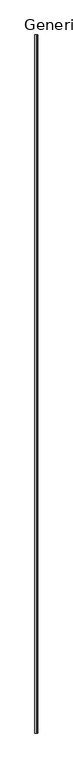
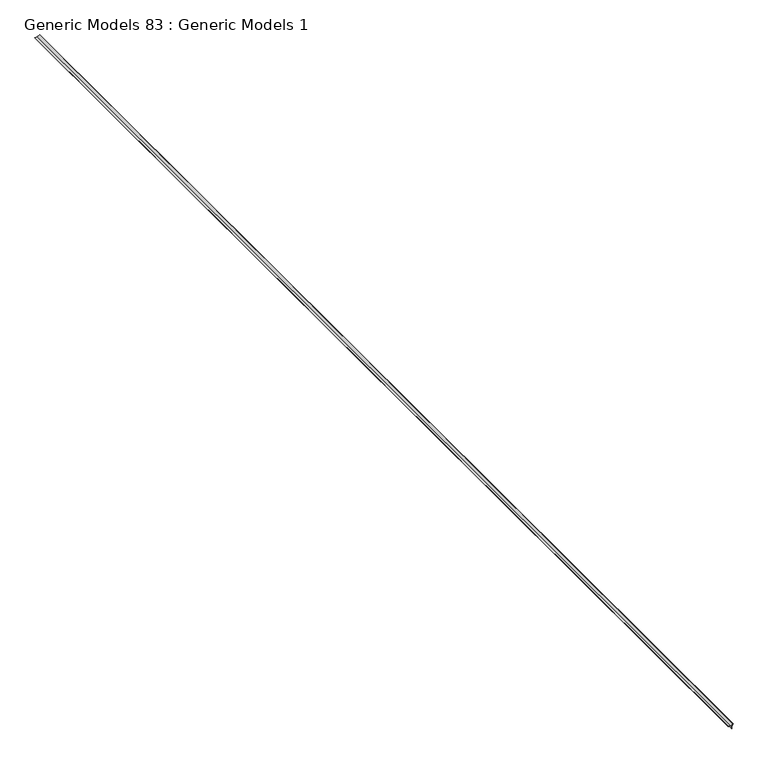
"""IFC4 building model written with IfcOpenShell, lengths in millimetres: proxy geometry, Generic Models 83 : Generic Models 1."""

from ifc_helpers import new_model, si_unit, point, frame, frame_2d, origin, place, context, project, spatial, polyline, circle_curve, trimmed, segment, composite_curve, outline, extrude, source, transform, mapped, element, save


def generic_models_83_generic_models_1_05889233(model_context):
    return source(origin(), model_context, "Body", "SweptSolid", [
        extrude(outline(composite_curve([segment(polyline([(127128.4926156, 9702.5518851), (127108.966, 9664.5263704), (127108.966, 9626.4263704), (127107.696, 9626.4263704), (127107.696, 9664.8333942), (127127.5962396, 9703.5864924), (127088.8431414, 9683.6862528), (127050.4361176, 9683.6862528), (127050.4361176, 9684.9562528), (127088.5361176, 9684.9562528), (127126.5616323, 9704.4828684)]), True, "CONTINUOUS"), segment(trimmed(circle_curve(frame_2d((127127.2167873, 9703.2070401)), 1.4342127), [point((127126.5616323, 9704.4828684))], [point((127128.4926156, 9702.5518851))], False, "CARTESIAN"), True, "CONTINUOUS")], self_intersect=False)), frame((0.0, -7068.1230338, 0.0), z_axis=(0.0, 1.0, 0.0), x_axis=(0.0, 0.0, 1.0)), (0.0, 0.0, 1.0), 19050.0),
    ])


if __name__ == "__main__":
    model = new_model("IFC4")
    model_context = context("Model", 3, world=origin())
    ifc_project = project(units=[si_unit("LENGTHUNIT", "METRE", prefix="MILLI")], contexts=[model_context])
    site = spatial("IfcSite", under=ifc_project)
    building = spatial("IfcBuilding", under=site)
    placement = place(None, origin())
    generic_models_83_generic_models_1_shape = generic_models_83_generic_models_1_05889233(model_context)
    element("IfcBuildingElementProxy", 1, Name="Generic Models 83 : Generic Models 1", ObjectType="Generic Models 83 : Generic Models 1", at=placement, inside=building, context=model_context, shape_type="MappedRepresentation", body=[
        mapped(generic_models_83_generic_models_1_shape, transform((0.0, 0.0, 0.0), x_axis=(1.0, 0.0, 0.0), y_axis=(0.0, 1.0, 0.0), z_axis=(0.0, 0.0, 1.0))),
    ])
    save(model, "model.ifc")

# Revit data of these elements
# Element 1 (IfcBuildingElementProxy, "Generic Models 83 : Generic Models 1")
#   Materials on its faces: "_CONTINUOUS 16 GA. COPPER CORNER BEAD"
# Materials
#   "_CONTINUOUS 16 GA. COPPER CORNER BEAD": class "Generic", colour RGB 253 192 103, transparency 0, Cost = 0
